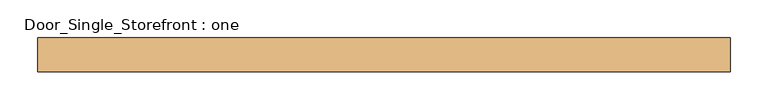
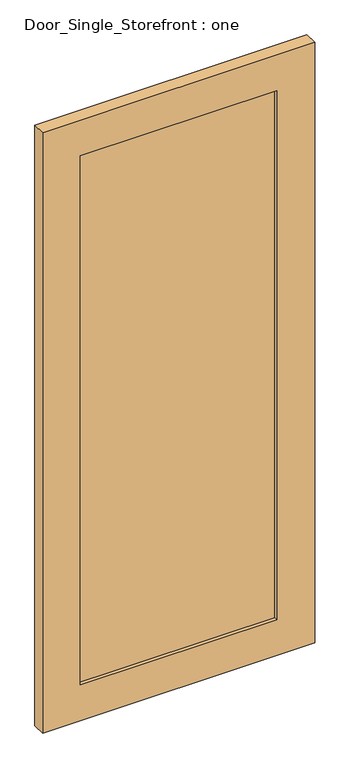
"""IFC4 building model written with IfcOpenShell, lengths in millimetres: door geometry, Door_Single_Storefront : one."""

from ifc_helpers import new_model, si_unit, frame, origin, place, context, project, spatial, polyline, outline, extrude, source, transform, mapped, element, save


def door_single_storefront_one_30533e89(model_context):
    return source(origin(), model_context, "Body", "SweptSolid", [
        extrude(outline(polyline([(330.2, -6.35), (-330.2, -6.35), (-330.2, 12.7), (330.2, 12.7), (330.2, -6.35)])), frame((0.0, 0.0, 127.0), z_axis=(0.0, 0.0, 1.0), x_axis=(1.0, 0.0, 0.0)), (0.0, 0.0, 1.0), 1879.6),
        extrude(outline(polyline([(2133.6, -457.2), (0.0, -457.2), (0.0, 457.2), (2133.6, 457.2), (2133.6, -457.2)]), holes=[polyline([(127.0, 330.2), (127.0, -330.2), (2006.6, -330.2), (2006.6, 330.2), (127.0, 330.2)])]), frame((0.0, -19.05, 0.0), z_axis=(0.0, 1.0, 0.0), x_axis=(0.0, 0.0, 1.0)), (0.0, 0.0, 1.0), 44.45),
    ])


if __name__ == "__main__":
    model = new_model("IFC4")
    model_context = context("Model", 3, world=origin())
    ifc_project = project(units=[si_unit("LENGTHUNIT", "METRE", prefix="MILLI")], contexts=[model_context])
    site = spatial("IfcSite", under=ifc_project)
    building = spatial("IfcBuilding", under=site)
    placement = place(None, origin())
    door_single_storefront_one_shape = door_single_storefront_one_30533e89(model_context)
    element("IfcDoor", 1, ObjectType="Door_Single_Storefront : one", at=placement, inside=building, context=model_context, shape_type="MappedRepresentation", body=[
        mapped(door_single_storefront_one_shape, transform((0.0, 0.0, 0.0), x_axis=(1.0, 0.0, 0.0), y_axis=(0.0, 1.0, 0.0), z_axis=(0.0, 0.0, 1.0))),
    ])
    save(model, "model.ifc")

# Revit data of these elements
# Type "Door_Single_Storefront : one"
#   Type Mark = "22"
#   Analytic Construction = "<None>"
#   Stile_Width = 0' - 5"
#   Door_Thickness = 0' - 1 3/4"
#   Door_Offset = 0' - 1"
#   Glass_Material = Glass
#   Frame_Material = Door - Panel
#   Function = (empty or 0)
# Element 1 (IfcDoor, "Door_Single_Storefront : one")
#   Materials on its faces: "Door - Panel", "Glass"
# Materials
#   "Glass": class "Glass", colour RGB 218 227 224, transparency 0.85, Description = "Soda Lime Glass", Cost = 0
#   "Door - Panel": class "Wood", colour RGB 114 82 51, transparency 0
